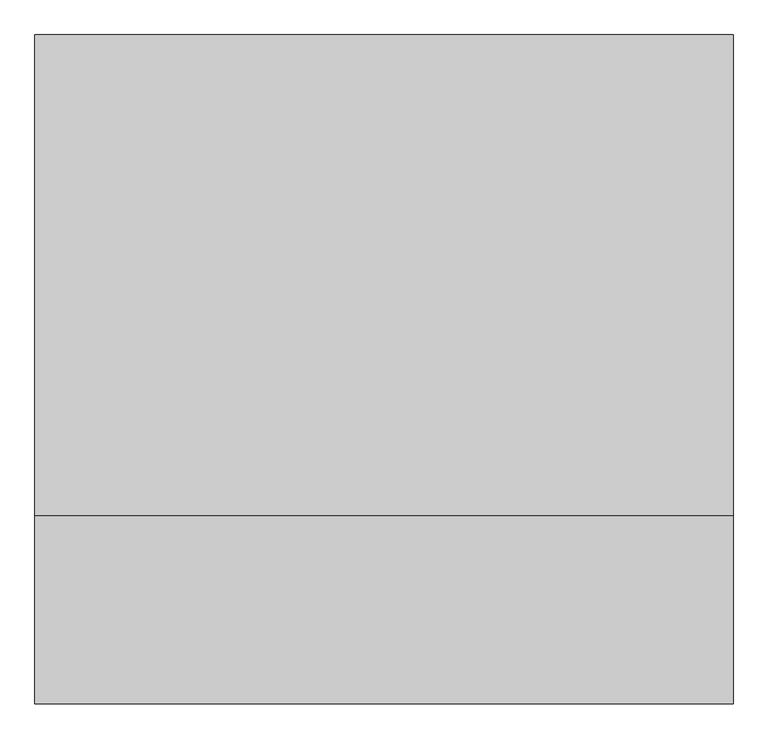
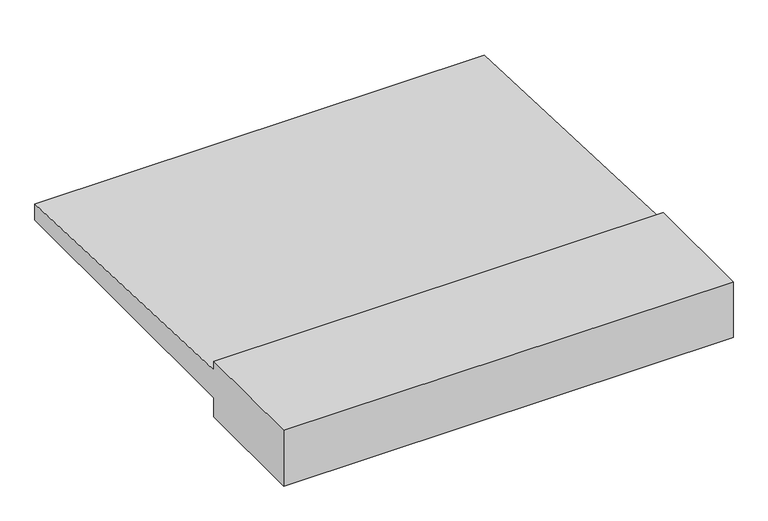
"""IFC4 building model written with IfcOpenShell, lengths in millimetres: plate geometry, 캐노피 : 캐노피."""

import ifcopenshell
import ifcopenshell.guid

model = None  # the IFC model being written
_history = None  # IfcOwnerHistory: only IFC2X3 demands one
_inside = {}  # id of a spatial element -> (the spatial element, [elements in it])
_under = {}  # id of a project, library or spatial element -> (it, [spatial elements below it])
_declared = {}  # id of a project -> (the project, [libraries it declares])
_typed = {}  # id of a type object -> (the type object, [elements of that type])
_made_of = {}  # id of a material, layer set ... -> (it, [elements and type objects made of it])


def new_model(schema):
    """Start an empty IFC model of exactly this schema.

    Asked for "IFC4X3", IfcOpenShell would pick the latest addendum, in which some entities
    have other attributes; the version numbers below select the first issue.
    IFC2X3 requires an IfcOwnerHistory on every rooted entity: one is made here for all.
    """
    global model, _history
    if schema == "IFC4X3":
        model = ifcopenshell.file(schema_version=(4, 3, 0, 0))
    else:
        model = ifcopenshell.file(schema=schema)
    _inside.clear()
    _under.clear()
    _declared.clear()
    _typed.clear()
    _made_of.clear()
    _history = None
    if model.schema == "IFC2X3":
        org = make("IfcOrganization", Name="unknown")
        user = make(
            "IfcPersonAndOrganization",
            ThePerson=make("IfcPerson", FamilyName="unknown"),
            TheOrganization=org,
        )
        app = make(
            "IfcApplication",
            ApplicationDeveloper=org,
            Version="unknown",
            ApplicationFullName="unknown",
            ApplicationIdentifier="unknown",
        )
        _history = make(
            "IfcOwnerHistory",
            OwningUser=user,
            OwningApplication=app,
            ChangeAction="ADDED",
            CreationDate=0,
        )
    return model


def make(cls, **values):
    """One entity of the class cls with the attributes given. An attribute that is None is left unset."""
    return model.create_entity(
        cls, **{name: value for name, value in values.items() if value is not None}
    )


def rooted(cls, **values):
    """An entity with a GlobalId (a new one), such as an element, a storey or a relation."""
    return make(cls, GlobalId=ifcopenshell.guid.new(), OwnerHistory=_history, **values)


def si_unit(unit_type, name, prefix=None):
    """IfcSIUnit, for example si_unit("LENGTHUNIT", "METRE", prefix="MILLI")."""
    return make("IfcSIUnit", UnitType=unit_type, Prefix=prefix, Name=name)


def assignment(units):
    """IfcUnitAssignment: the units of a project."""
    return None if units is None else make("IfcUnitAssignment", Units=units)


def point(xyz):
    """IfcCartesianPoint."""
    return None if xyz is None else make("IfcCartesianPoint", Coordinates=xyz)


def direction(xyz):
    """IfcDirection."""
    return None if xyz is None else make("IfcDirection", DirectionRatios=xyz)


def frame(location, z_axis=None, x_axis=None):
    """IfcAxis2Placement3D, a coordinate frame: its origin and axes. An axis left out is left unset."""
    return make(
        "IfcAxis2Placement3D",
        Location=point(location),
        Axis=direction(z_axis),
        RefDirection=direction(x_axis),
    )


def origin():
    """The frame at (0, 0, 0) with its axes left unset."""
    return frame((0.0, 0.0, 0.0))


def place(relative_to, where):
    """IfcLocalPlacement: puts the frame where relative to a parent placement (None: the world)."""
    return make(
        "IfcLocalPlacement", PlacementRelTo=relative_to, RelativePlacement=where
    )


def context(
    kind, dimensions, precision=None, world=None, true_north=None, identifier=None
):
    """IfcGeometricRepresentationContext, for example the 3D "Model" context."""
    return make(
        "IfcGeometricRepresentationContext",
        ContextIdentifier=identifier,
        ContextType=kind,
        CoordinateSpaceDimension=dimensions,
        Precision=precision,
        WorldCoordinateSystem=world,
        TrueNorth=true_north,
    )


def project(units=None, contexts=None):
    """IfcProject with its units and contexts."""
    return rooted(
        "IfcProject",
        Name="project",
        RepresentationContexts=contexts,
        UnitsInContext=assignment(units),
    )


def spatial(cls, under=None, at=None, **own):
    """A site, building, storey or space (cls), placed at a placement, below another one or the project."""
    s = rooted(cls, ObjectPlacement=at, **own)
    if under is not None:
        _under.setdefault(under.id(), (under, []))[1].append(s)
    return s


def polyline(points):
    """IfcPolyline through the points."""
    return make("IfcPolyline", Points=[point(p) for p in points])


def outline(outer, holes=None, kind="AREA"):
    """IfcArbitraryClosedProfileDef: a profile drawn as a closed curve; with holes, ...WithVoids."""
    if holes is None:
        return make("IfcArbitraryClosedProfileDef", ProfileType=kind, OuterCurve=outer)
    return make(
        "IfcArbitraryProfileDefWithVoids",
        ProfileType=kind,
        OuterCurve=outer,
        InnerCurves=holes,
    )


def extrude(swept, where, along, depth):
    """IfcExtrudedAreaSolid: the profile swept, set in the frame where, extruded along a direction by depth."""
    return make(
        "IfcExtrudedAreaSolid",
        SweptArea=swept,
        Position=where,
        ExtrudedDirection=direction(along),
        Depth=depth,
    )


def shape(context_of_items, identifier, shape_type, items):
    """IfcShapeRepresentation: the items that make up one representation, for example the "Body"."""
    return make(
        "IfcShapeRepresentation",
        ContextOfItems=context_of_items,
        RepresentationIdentifier=identifier,
        RepresentationType=shape_type,
        Items=items,
    )


def source(mapping_origin, context_of_items, identifier, shape_type, items):
    """IfcRepresentationMap: a shape defined once, which mapped items show again and again."""
    return make(
        "IfcRepresentationMap",
        MappingOrigin=mapping_origin,
        MappedRepresentation=shape(context_of_items, identifier, shape_type, items),
    )


def transform(
    local_origin,
    x_axis=None,
    y_axis=None,
    z_axis=None,
    scale=None,
    scale2=None,
    scale3=None,
    uniform=True,
):
    """IfcCartesianTransformationOperator3D, or its non-uniform kind. x_axis, y_axis, z_axis: its Axis1, 2, 3."""
    if uniform:
        return make(
            "IfcCartesianTransformationOperator3D",
            Axis1=direction(x_axis),
            Axis2=direction(y_axis),
            LocalOrigin=point(local_origin),
            Scale=scale,
            Axis3=direction(z_axis),
        )
    return make(
        "IfcCartesianTransformationOperator3DnonUniform",
        Axis1=direction(x_axis),
        Axis2=direction(y_axis),
        LocalOrigin=point(local_origin),
        Scale=scale,
        Axis3=direction(z_axis),
        Scale2=scale2,
        Scale3=scale3,
    )


def mapped(mapping_source, mapping_target):
    """IfcMappedItem: shows the shape of a source again, moved by a transform."""
    return make(
        "IfcMappedItem", MappingSource=mapping_source, MappingTarget=mapping_target
    )


def made_of(thing, what):
    """Note that an element or type object is made of a material, layer set ...; save() writes the relation."""
    if what is not None:
        _made_of.setdefault(what.id(), (what, []))[1].append(thing)
    return thing


def element(
    cls,
    number,
    at=None,
    inside=None,
    cuts=None,
    type_object=None,
    material=None,
    context=None,
    identifier="Body",
    shape_type=None,
    held_by="IfcProductDefinitionShape",
    body=None,
    shapes=None,
    **own,
):
    """One element of the class cls, such as IfcWall. Its Tag is "e" and its number.

    at: its placement. inside: the storey or other place that contains it. cuts: it is an
    opening in that element (IfcRelVoidsElement). A single representation is given by context,
    identifier, shape_type and body (its items); several are given by shapes. held_by: the class
    of the entity that holds the representations. save() writes the other relations.
    """
    e = rooted(cls, Tag="e%d" % number, ObjectPlacement=at, **own)
    if body is not None:
        shapes = [shape(context, identifier, shape_type, body)]
    if shapes is not None:
        e.Representation = make(held_by, Representations=shapes)
    if inside is not None:
        _inside.setdefault(inside.id(), (inside, []))[1].append(e)
    if cuts is not None:
        rooted(
            "IfcRelVoidsElement", RelatingBuildingElement=cuts, RelatedOpeningElement=e
        )
    if type_object is not None:
        _typed.setdefault(type_object.id(), (type_object, []))[1].append(e)
    return made_of(e, material)


def aggregate(whole, parts):
    """IfcRelAggregates: a whole, such as a stair, and the parts it consists of."""
    return rooted("IfcRelAggregates", RelatingObject=whole, RelatedObjects=parts)


def save(model, path):
    """Write the relations noted so far, then the file.

    IfcRelAggregates (storeys below a building ...), IfcRelContainedInSpatialStructure (elements
    in a storey), IfcRelDefinesByType, IfcRelAssociatesMaterial and IfcRelDeclares: one each for
    every whole, place, type object, material and project.
    """
    for whole, parts in _under.values():
        aggregate(whole, parts)
    for where, things in _inside.values():
        rooted(
            "IfcRelContainedInSpatialStructure",
            RelatedElements=things,
            RelatingStructure=where,
        )
    for kind, things in _typed.values():
        rooted("IfcRelDefinesByType", RelatedObjects=things, RelatingType=kind)
    for what, things in _made_of.values():
        rooted("IfcRelAssociatesMaterial", RelatedObjects=things, RelatingMaterial=what)
    for by, libraries in _declared.values():
        rooted("IfcRelDeclares", RelatingContext=by, RelatedDefinitions=libraries)
    model.write(path)


def plate_1abda111(model_context):
    return source(origin(), model_context, "Body", "SweptSolid", [
        extrude(outline(polyline([(-195.0, 800.0), (-195.0, 990.0), (195.0, 990.0), (195.0, 960.0), (1195.0, 920.0), (1195.0, 865.0), (195.0, 865.0), (195.0, 800.0), (-195.0, 800.0)])), frame((-725.0, 0.0, 0.0), z_axis=(1.0, 0.0, 0.0), x_axis=(0.0, 1.0, 0.0)), (0.0, 0.0, 1.0), 1450.0),
    ])


if __name__ == "__main__":
    model = new_model("IFC4")
    model_context = context("Model", 3, world=origin())
    ifc_project = project(units=[si_unit("LENGTHUNIT", "METRE", prefix="MILLI")], contexts=[model_context])
    site = spatial("IfcSite", under=ifc_project)
    building = spatial("IfcBuilding", under=site)
    placement = place(None, origin())
    plate_shape = plate_1abda111(model_context)
    element("IfcPlate", 1, ObjectType="캐노피 : 캐노피", at=placement, inside=building, context=model_context, shape_type="MappedRepresentation", body=[
        mapped(plate_shape, transform((0.0, 0.0, 0.0), x_axis=(1.0, 0.0, 0.0), y_axis=(0.0, 1.0, 0.0), z_axis=(0.0, 0.0, 1.0))),
    ])
    save(model, "model.ifc")

# Revit data of these elements
# Type "캐노피 : 캐노피"
#   Type Mark = "203"
#   Width = 1450 mm
#   Height = 190 mm
#   돌출길이 = 1000 mm
#   Default Sill Height = 800 mm
#   Wall Closure = (empty or 0)
